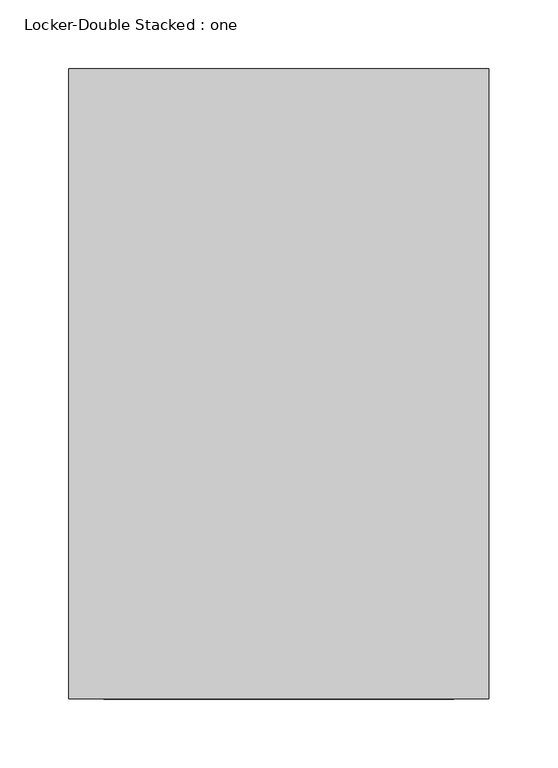
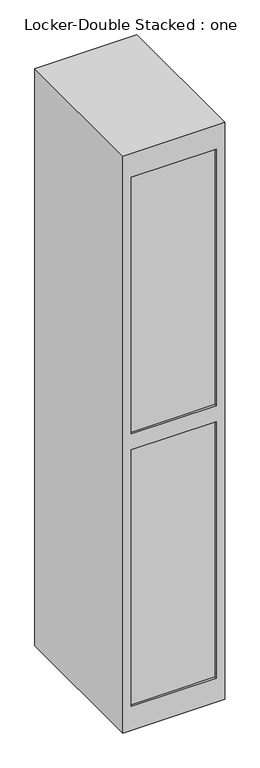
"""IFC4 building model written with IfcOpenShell, lengths in millimetres: furniture geometry, Locker-Double Stacked : one."""

from ifc_helpers import new_model, si_unit, origin, place, context, project, spatial, faceted_brep, source, transform, mapped, element, save


def locker_double_stacked_one_5313e0f4(model_context):
    return source(origin(), model_context, "Body", "Brep", [
        faceted_brep([(152.4, -228.6, 1828.8), (152.4, 228.6, 1828.8), (-152.4, 228.6, 1828.8), (-152.4, -228.6, 1828.8), (152.4, -228.6, 0.0), (-152.4, -228.6, 0.0), (-152.4, 228.6, 0.0), (152.4, 228.6, 0.0), (127.0, -228.6, 889.0), (127.0, -228.6, 76.2), (-127.0, -228.6, 76.2), (-127.0, -228.6, 889.0), (-127.0, -228.6, 1752.6), (127.0, -228.6, 1752.6), (127.0, -228.6, 939.8), (-127.0, -228.6, 939.8), (127.0, -222.25, 76.2), (127.0, -222.25, 889.0), (-127.0, -222.25, 889.0), (-127.0, -222.25, 76.2), (127.0, -222.25, 1752.6), (-127.0, -222.25, 1752.6), (-127.0, -222.25, 939.8), (127.0, -222.25, 939.8)], [[[0, 1, 2, 3]], [[4, 5, 6, 7]], [[1, 0, 4, 7]], [[2, 1, 7, 6]], [[3, 2, 6, 5]], [[0, 3, 5, 4], [8, 9, 10, 11], [12, 13, 14, 15]], [[16, 17, 18, 19]], [[17, 16, 9, 8]], [[18, 17, 8, 11]], [[19, 18, 11, 10]], [[16, 19, 10, 9]], [[20, 21, 22, 23]], [[21, 20, 13, 12]], [[22, 21, 12, 15]], [[23, 22, 15, 14]], [[20, 23, 14, 13]]]),
    ])


if __name__ == "__main__":
    model = new_model("IFC4")
    model_context = context("Model", 3, world=origin())
    ifc_project = project(units=[si_unit("LENGTHUNIT", "METRE", prefix="MILLI")], contexts=[model_context])
    site = spatial("IfcSite", under=ifc_project)
    building = spatial("IfcBuilding", under=site)
    placement = place(None, origin())
    locker_double_stacked_one_shape = locker_double_stacked_one_5313e0f4(model_context)
    element("IfcFurniture", 1, ObjectType="Locker-Double Stacked : one", at=placement, inside=building, context=model_context, shape_type="MappedRepresentation", body=[
        mapped(locker_double_stacked_one_shape, transform((0.0, 0.0, 0.0), x_axis=(1.0, 0.0, 0.0), y_axis=(0.0, 1.0, 0.0), z_axis=(0.0, 0.0, 1.0))),
    ])
    save(model, "model.ifc")

# Revit data of these elements
# Type "Locker-Double Stacked : one"
#   Keynote = "M10511300.01"
#   Assembly Code = "E2010"
#   Depth = 1' - 6"
#   Height = 6' - 0"
#   Width = 1' - 0"
#   Material = LOCKERS
# Element 1 (IfcFurniture, "Locker-Double Stacked : one")
#   Materials on its faces: "LOCKERS"
# Materials
#   "LOCKERS": class "Metal", colour RGB 181 181 181, transparency 0, Cost = 0
